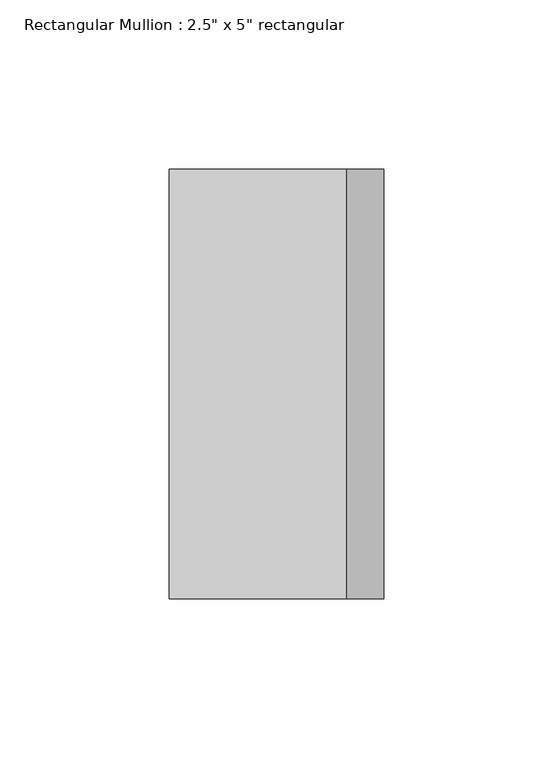
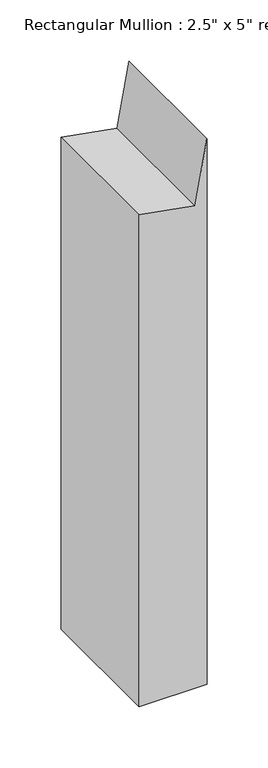
"""IFC4 building model written with IfcOpenShell, lengths in millimetres: member geometry."""

from ifc_helpers import new_model, si_unit, frame, origin, place, context, project, spatial, polyline, outline, extrude, source, transform, mapped, element, save


def member_2b5633e6(model_context):
    return source(origin(), model_context, "Body", "SweptSolid", [
        extrude(outline(polyline([(0.0, 0.0), (-62.5352923, -11.0266593), (-53.2828266, -63.5), (-541.6285548, -63.5), (-541.6285548, 0.0), (0.0, 0.0)])), frame((0.0, -63.5, 0.0), z_axis=(0.0, 1.0, 0.0), x_axis=(0.0, 0.0, 1.0)), (0.0, 0.0, 1.0), 127.0),
    ])


if __name__ == "__main__":
    model = new_model("IFC4")
    model_context = context("Model", 3, world=origin())
    ifc_project = project(units=[si_unit("LENGTHUNIT", "METRE", prefix="MILLI")], contexts=[model_context])
    site = spatial("IfcSite", under=ifc_project)
    building = spatial("IfcBuilding", under=site)
    placement = place(None, origin())
    member_shape = member_2b5633e6(model_context)
    element("IfcMember", 1, ObjectType="Rectangular Mullion : 2.5\" x 5\" rectangular", at=placement, inside=building, context=model_context, shape_type="MappedRepresentation", body=[
        mapped(member_shape, transform((0.0, 0.0, 0.0), x_axis=(1.0, 0.0, 0.0), y_axis=(0.0, 1.0, 0.0), z_axis=(0.0, 0.0, 1.0))),
    ])
    save(model, "model.ifc")

# Revit data of these elements
# Type "Rectangular Mullion : 2.5\" x 5\" rectangular"
#   built-in parameter 1007304 = 0.416667 (stored number, unit not read)
#   built-in parameter 1007301 = 0.104167 (stored number, unit not read)
#   built-in parameter 1007300 = 0.104167 (stored number, unit not read)
# Element 1 (IfcMember, "Rectangular Mullion : 2.5\" x 5\" rectangular")
#   Materials on its faces: "Black Mullions"
# Materials
#   "Black Mullions": class "Wood", colour RGB 0 0 0, transparency 0, Cost = 0
